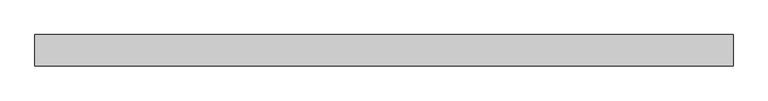
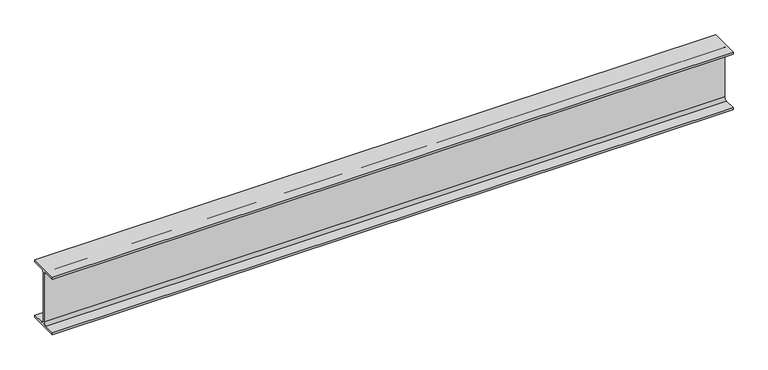
"""IFC4 building model written with IfcOpenShell, lengths in millimetres: beam geometry, 0912_Steel Framing_H-KSD3502 : H_SB_ASB_H-250x125x6x9."""

from ifc_helpers import new_model, si_unit, point, frame, frame_2d, origin, place, context, project, spatial, polyline, circle_curve, trimmed, segment, composite_curve, outline, extrude, source, transform, mapped, element, save


def beam_8986b571(model_context):
    return source(origin(), model_context, "Body", "SweptSolid", [
        extrude(outline(composite_curve([segment(polyline([(62.5, -116.0), (62.5, -125.0), (-62.5, -125.0), (-62.5, -116.0), (-15.0, -116.0)]), True, "CONTINUOUS"), segment(trimmed(circle_curve(frame_2d((-15.0, -104.0)), 12.0), [point((-15.0, -116.0))], [point((-3.0, -104.0))], True, "CARTESIAN"), True, "CONTINUOUS"), segment(polyline([(-3.0, -104.0), (-3.0, 104.0)]), True, "CONTINUOUS"), segment(trimmed(circle_curve(frame_2d((-15.0, 104.0)), 12.0), [point((-3.0, 104.0))], [point((-15.0, 116.0))], True, "CARTESIAN"), True, "CONTINUOUS"), segment(polyline([(-15.0, 116.0), (-62.5, 116.0), (-62.5, 125.0), (62.5, 125.0), (62.5, 116.0), (15.0, 116.0)]), True, "CONTINUOUS"), segment(trimmed(circle_curve(frame_2d((15.0, 104.0)), 12.0), [point((15.0, 116.0))], [point((3.0, 104.0))], True, "CARTESIAN"), True, "CONTINUOUS"), segment(polyline([(3.0, 104.0), (3.0, -104.0)]), True, "CONTINUOUS"), segment(trimmed(circle_curve(frame_2d((15.0, -104.0)), 12.0), [point((3.0, -104.0))], [point((15.0, -116.0))], True, "CARTESIAN"), True, "CONTINUOUS"), segment(polyline([(15.0, -116.0), (62.5, -116.0)]), True, "CONTINUOUS")], self_intersect=False)), frame((-1382.3488581, 0.0, 0.0), z_axis=(1.0, 0.0, 0.0), x_axis=(0.0, 1.0, 0.0)), (0.0, 0.0, 1.0), 2794.6488581),
    ])


if __name__ == "__main__":
    model = new_model("IFC4")
    model_context = context("Model", 3, world=origin())
    ifc_project = project(units=[si_unit("LENGTHUNIT", "METRE", prefix="MILLI")], contexts=[model_context])
    site = spatial("IfcSite", under=ifc_project)
    building = spatial("IfcBuilding", under=site)
    placement = place(None, origin())
    beam_shape = beam_8986b571(model_context)
    element("IfcBeam", 1, ObjectType="0912_Steel Framing_H-KSD3502 : H_SB_ASB_H-250x125x6x9", at=placement, inside=building, context=model_context, shape_type="MappedRepresentation", body=[
        mapped(beam_shape, transform((0.0, 0.0, 0.0), x_axis=(1.0, 0.0, 0.0), y_axis=(0.0, 1.0, 0.0), z_axis=(0.0, 0.0, 1.0))),
    ])
    save(model, "model.ifc")

# Revit data of these elements
# Type "0912_Steel Framing_H-KSD3502 : H_SB_ASB_H-250x125x6x9"
#   H_WM Code_1 = "S01AA003-00001 | Main Steel Structure Fabrication Work | Shelter/Building | Light Steel - Standard (30KG/M>Weight) | Material: (   )"
#   H_WM Code_2 = "S03AA029-00001 | Main Steel Structure Erection Work | Shelter/Building | Light Steel (30KG/M>Weight) | Material: (   )"
#   H_WM Code_3 = "S01AA010-00001 | Main Steel Structure Fabrication Work | Shelter/Building | Steel Painting/Coating | for Non-Fireproofed Steel Surface, Surface Preparation, Primer, Second & Final Coat | Material: (   )"
#   H_Q'ty Cal Type Tag = "SB-Q2"
#   Width = 12.5 cm
#   Web Thickness = 0.6 cm
#   Web Fillet = 1.2 cm
#   Warping Constant = 42539.8 cm⁶
#   W = 0
#   Torsional Moment of Inertia = 7.8102 cm⁴
#   Section Area = 37.66 cm²
#   Plastic Modulus weak axis = 73.1 cm³
#   Plastic Modulus strong axis = 366.0 cm³
#   Perimeter = 0.97 m²/m
#   Nominal Weight = 29.60 kgf/m
#   Moment of Inertia weak axis = 294.00 cm⁴
#   Moment of Inertia strong axis = 4050.00 cm⁴
#   Height = 25.0 cm
#   Flange Thickness = 0.9 cm
#   Elastic Modulus weak axis = 47.0 cm³
#   Elastic Modulus strong axis = 324.0 cm³
#   Centroid Vertical = 12.5 cm
#   Centroid Horizontal = 6.25 cm
#   Ix = 40500000
#   Length [instance default] = 1.5240 m
#   Zx = 366000
#   b = 0.1250 m
#   h = 0.2500 m
#   r = 0.0120 m
#   s = 0.0060 m
#   t = 0.0090 m
#   A = 0.003766 m²
#   Structural Material [instance default] = Steel, 45-345
#   Assembly Code = ""
# Element 1 (IfcBeam, "0912_Steel Framing_H-KSD3502 : H_SB_ASB_H-250x125x6x9")
#   Structural Material = none
# Materials
#   "Steel, 45-345": class "Metal", colour RGB 189 187 185, transparency 0, Description = "Steel 345 MPa", Cost = 0
